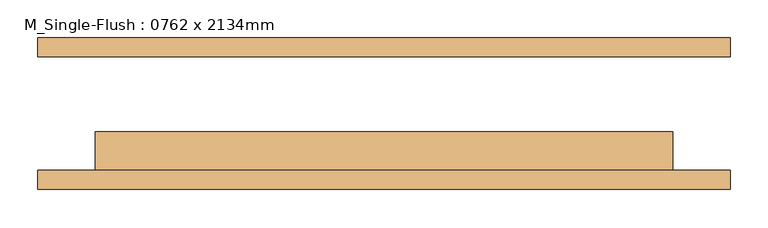
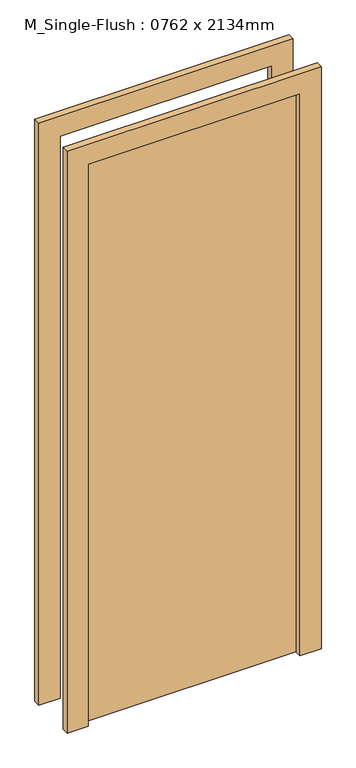
"""IFC4 building model written with IfcOpenShell, lengths in millimetres: door geometry, M_Single-Flush : 0762 x 2134mm."""

import ifcopenshell
import ifcopenshell.guid

model = None  # the IFC model being written
_history = None  # IfcOwnerHistory: only IFC2X3 demands one
_inside = {}  # id of a spatial element -> (the spatial element, [elements in it])
_under = {}  # id of a project, library or spatial element -> (it, [spatial elements below it])
_declared = {}  # id of a project -> (the project, [libraries it declares])
_typed = {}  # id of a type object -> (the type object, [elements of that type])
_made_of = {}  # id of a material, layer set ... -> (it, [elements and type objects made of it])


def new_model(schema):
    """Start an empty IFC model of exactly this schema.

    Asked for "IFC4X3", IfcOpenShell would pick the latest addendum, in which some entities
    have other attributes; the version numbers below select the first issue.
    IFC2X3 requires an IfcOwnerHistory on every rooted entity: one is made here for all.
    """
    global model, _history
    if schema == "IFC4X3":
        model = ifcopenshell.file(schema_version=(4, 3, 0, 0))
    else:
        model = ifcopenshell.file(schema=schema)
    _inside.clear()
    _under.clear()
    _declared.clear()
    _typed.clear()
    _made_of.clear()
    _history = None
    if model.schema == "IFC2X3":
        org = make("IfcOrganization", Name="unknown")
        user = make(
            "IfcPersonAndOrganization",
            ThePerson=make("IfcPerson", FamilyName="unknown"),
            TheOrganization=org,
        )
        app = make(
            "IfcApplication",
            ApplicationDeveloper=org,
            Version="unknown",
            ApplicationFullName="unknown",
            ApplicationIdentifier="unknown",
        )
        _history = make(
            "IfcOwnerHistory",
            OwningUser=user,
            OwningApplication=app,
            ChangeAction="ADDED",
            CreationDate=0,
        )
    return model


def make(cls, **values):
    """One entity of the class cls with the attributes given. An attribute that is None is left unset."""
    return model.create_entity(
        cls, **{name: value for name, value in values.items() if value is not None}
    )


def rooted(cls, **values):
    """An entity with a GlobalId (a new one), such as an element, a storey or a relation."""
    return make(cls, GlobalId=ifcopenshell.guid.new(), OwnerHistory=_history, **values)


def si_unit(unit_type, name, prefix=None):
    """IfcSIUnit, for example si_unit("LENGTHUNIT", "METRE", prefix="MILLI")."""
    return make("IfcSIUnit", UnitType=unit_type, Prefix=prefix, Name=name)


def assignment(units):
    """IfcUnitAssignment: the units of a project."""
    return None if units is None else make("IfcUnitAssignment", Units=units)


def point(xyz):
    """IfcCartesianPoint."""
    return None if xyz is None else make("IfcCartesianPoint", Coordinates=xyz)


def direction(xyz):
    """IfcDirection."""
    return None if xyz is None else make("IfcDirection", DirectionRatios=xyz)


def frame(location, z_axis=None, x_axis=None):
    """IfcAxis2Placement3D, a coordinate frame: its origin and axes. An axis left out is left unset."""
    return make(
        "IfcAxis2Placement3D",
        Location=point(location),
        Axis=direction(z_axis),
        RefDirection=direction(x_axis),
    )


def origin():
    """The frame at (0, 0, 0) with its axes left unset."""
    return frame((0.0, 0.0, 0.0))


def origin_with_axes():
    """The frame at (0, 0, 0) with the z axis (0, 0, 1) and the x axis (1, 0, 0) written out."""
    return frame((0.0, 0.0, 0.0), z_axis=(0.0, 0.0, 1.0), x_axis=(1.0, 0.0, 0.0))


def place(relative_to, where):
    """IfcLocalPlacement: puts the frame where relative to a parent placement (None: the world)."""
    return make(
        "IfcLocalPlacement", PlacementRelTo=relative_to, RelativePlacement=where
    )


def context(
    kind, dimensions, precision=None, world=None, true_north=None, identifier=None
):
    """IfcGeometricRepresentationContext, for example the 3D "Model" context."""
    return make(
        "IfcGeometricRepresentationContext",
        ContextIdentifier=identifier,
        ContextType=kind,
        CoordinateSpaceDimension=dimensions,
        Precision=precision,
        WorldCoordinateSystem=world,
        TrueNorth=true_north,
    )


def project(units=None, contexts=None):
    """IfcProject with its units and contexts."""
    return rooted(
        "IfcProject",
        Name="project",
        RepresentationContexts=contexts,
        UnitsInContext=assignment(units),
    )


def spatial(cls, under=None, at=None, **own):
    """A site, building, storey or space (cls), placed at a placement, below another one or the project."""
    s = rooted(cls, ObjectPlacement=at, **own)
    if under is not None:
        _under.setdefault(under.id(), (under, []))[1].append(s)
    return s


def polyline(points):
    """IfcPolyline through the points."""
    return make("IfcPolyline", Points=[point(p) for p in points])


def outline(outer, holes=None, kind="AREA"):
    """IfcArbitraryClosedProfileDef: a profile drawn as a closed curve; with holes, ...WithVoids."""
    if holes is None:
        return make("IfcArbitraryClosedProfileDef", ProfileType=kind, OuterCurve=outer)
    return make(
        "IfcArbitraryProfileDefWithVoids",
        ProfileType=kind,
        OuterCurve=outer,
        InnerCurves=holes,
    )


def extrude(swept, where, along, depth):
    """IfcExtrudedAreaSolid: the profile swept, set in the frame where, extruded along a direction by depth."""
    return make(
        "IfcExtrudedAreaSolid",
        SweptArea=swept,
        Position=where,
        ExtrudedDirection=direction(along),
        Depth=depth,
    )


def shape(context_of_items, identifier, shape_type, items):
    """IfcShapeRepresentation: the items that make up one representation, for example the "Body"."""
    return make(
        "IfcShapeRepresentation",
        ContextOfItems=context_of_items,
        RepresentationIdentifier=identifier,
        RepresentationType=shape_type,
        Items=items,
    )


def source(mapping_origin, context_of_items, identifier, shape_type, items):
    """IfcRepresentationMap: a shape defined once, which mapped items show again and again."""
    return make(
        "IfcRepresentationMap",
        MappingOrigin=mapping_origin,
        MappedRepresentation=shape(context_of_items, identifier, shape_type, items),
    )


def transform(
    local_origin,
    x_axis=None,
    y_axis=None,
    z_axis=None,
    scale=None,
    scale2=None,
    scale3=None,
    uniform=True,
):
    """IfcCartesianTransformationOperator3D, or its non-uniform kind. x_axis, y_axis, z_axis: its Axis1, 2, 3."""
    if uniform:
        return make(
            "IfcCartesianTransformationOperator3D",
            Axis1=direction(x_axis),
            Axis2=direction(y_axis),
            LocalOrigin=point(local_origin),
            Scale=scale,
            Axis3=direction(z_axis),
        )
    return make(
        "IfcCartesianTransformationOperator3DnonUniform",
        Axis1=direction(x_axis),
        Axis2=direction(y_axis),
        LocalOrigin=point(local_origin),
        Scale=scale,
        Axis3=direction(z_axis),
        Scale2=scale2,
        Scale3=scale3,
    )


def mapped(mapping_source, mapping_target):
    """IfcMappedItem: shows the shape of a source again, moved by a transform."""
    return make(
        "IfcMappedItem", MappingSource=mapping_source, MappingTarget=mapping_target
    )


def made_of(thing, what):
    """Note that an element or type object is made of a material, layer set ...; save() writes the relation."""
    if what is not None:
        _made_of.setdefault(what.id(), (what, []))[1].append(thing)
    return thing


def element(
    cls,
    number,
    at=None,
    inside=None,
    cuts=None,
    type_object=None,
    material=None,
    context=None,
    identifier="Body",
    shape_type=None,
    held_by="IfcProductDefinitionShape",
    body=None,
    shapes=None,
    **own,
):
    """One element of the class cls, such as IfcWall. Its Tag is "e" and its number.

    at: its placement. inside: the storey or other place that contains it. cuts: it is an
    opening in that element (IfcRelVoidsElement). A single representation is given by context,
    identifier, shape_type and body (its items); several are given by shapes. held_by: the class
    of the entity that holds the representations. save() writes the other relations.
    """
    e = rooted(cls, Tag="e%d" % number, ObjectPlacement=at, **own)
    if body is not None:
        shapes = [shape(context, identifier, shape_type, body)]
    if shapes is not None:
        e.Representation = make(held_by, Representations=shapes)
    if inside is not None:
        _inside.setdefault(inside.id(), (inside, []))[1].append(e)
    if cuts is not None:
        rooted(
            "IfcRelVoidsElement", RelatingBuildingElement=cuts, RelatedOpeningElement=e
        )
    if type_object is not None:
        _typed.setdefault(type_object.id(), (type_object, []))[1].append(e)
    return made_of(e, material)


def aggregate(whole, parts):
    """IfcRelAggregates: a whole, such as a stair, and the parts it consists of."""
    return rooted("IfcRelAggregates", RelatingObject=whole, RelatedObjects=parts)


def save(model, path):
    """Write the relations noted so far, then the file.

    IfcRelAggregates (storeys below a building ...), IfcRelContainedInSpatialStructure (elements
    in a storey), IfcRelDefinesByType, IfcRelAssociatesMaterial and IfcRelDeclares: one each for
    every whole, place, type object, material and project.
    """
    for whole, parts in _under.values():
        aggregate(whole, parts)
    for where, things in _inside.values():
        rooted(
            "IfcRelContainedInSpatialStructure",
            RelatedElements=things,
            RelatingStructure=where,
        )
    for kind, things in _typed.values():
        rooted("IfcRelDefinesByType", RelatedObjects=things, RelatingType=kind)
    for what, things in _made_of.values():
        rooted("IfcRelAssociatesMaterial", RelatedObjects=things, RelatingMaterial=what)
    for by, libraries in _declared.values():
        rooted("IfcRelDeclares", RelatingContext=by, RelatedDefinitions=libraries)
    model.write(path)


def m_single_flush_0762_x_2134mm_8c18b9de(model_context):
    return source(origin(), model_context, "Body", "SweptSolid", [
        extrude(outline(polyline([(2210.0, -457.0), (0.0, -457.0), (0.0, -381.0), (2134.0, -381.0), (2134.0, 381.0), (0.0, 381.0), (0.0, 457.0), (2210.0, 457.0), (2210.0, -457.0)])), frame((0.0, -100.0, 0.0), z_axis=(0.0, 1.0, 0.0), x_axis=(0.0, 0.0, 1.0)), (0.0, 0.0, 1.0), 25.0),
        extrude(outline(polyline([(2210.0, 457.0), (2210.0, -457.0), (0.0, -457.0), (0.0, -381.0), (2134.0, -381.0), (2134.0, 381.0), (0.0, 381.0), (0.0, 457.0), (2210.0, 457.0)])), frame((0.0, 75.0, 0.0), z_axis=(0.0, 1.0, 0.0), x_axis=(0.0, 0.0, 1.0)), (0.0, 0.0, 1.0), 25.0),
        extrude(outline(polyline([(381.0, -24.0), (381.0, -75.0), (-381.0, -75.0), (-381.0, -24.0), (381.0, -24.0)])), origin_with_axes(), (0.0, 0.0, 1.0), 2134.0),
    ])


if __name__ == "__main__":
    model = new_model("IFC4")
    model_context = context("Model", 3, world=origin())
    ifc_project = project(units=[si_unit("LENGTHUNIT", "METRE", prefix="MILLI")], contexts=[model_context])
    site = spatial("IfcSite", under=ifc_project)
    building = spatial("IfcBuilding", under=site)
    placement = place(None, origin())
    m_single_flush_0762_x_2134mm_shape = m_single_flush_0762_x_2134mm_8c18b9de(model_context)
    element("IfcDoor", 1, ObjectType="M_Single-Flush : 0762 x 2134mm", at=placement, inside=building, context=model_context, shape_type="MappedRepresentation", body=[
        mapped(m_single_flush_0762_x_2134mm_shape, transform((0.0, 0.0, 0.0), x_axis=(1.0, 0.0, 0.0), y_axis=(0.0, 1.0, 0.0), z_axis=(0.0, 0.0, 1.0))),
    ])
    save(model, "model.ifc")

# Revit data of these elements
# Type "M_Single-Flush : 0762 x 2134mm"
#   Type Mark = "16"
#   Construction Type Id = "MDOOR"
#   Analytic Construction = "Metal"
#   Thickness = 5.1 cm
#   Thermal Resistance (R) = 0.270117 (m²·K)/W
#   Heat Transfer Coefficient (U) = 3.7021 W/(m²·K)
#   Height = 213.4 cm
#   Trim Projection Ext = 2.5 cm
#   Trim Projection Int = 2.5 cm
#   Trim Width = 7.6 cm
#   Width = 76.2 cm
#   Define Thermal Properties by = 1
#   Define Thermal Properties by = 1
#   Door Material = Door - Panel
#   Frame Material = Door - Frame
#   Visual Light Transmittance = 0
#   Solar Heat Gain Coefficient = 0
#   Function = (empty or 0)
#   Wall Closure = (empty or 0)
# Element 1 (IfcDoor, "M_Single-Flush : 0762 x 2134mm")
#   Materials on its faces: "Door - Frame", "Door - Panel"
# Materials
#   "Door - Panel": class "Wood", colour RGB 210 159 95, transparency 0, Cost = 0
#   "Door - Frame": class "Miscellaneous", colour RGB 118 70 51, transparency 0, Cost = 0
